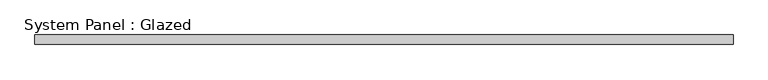
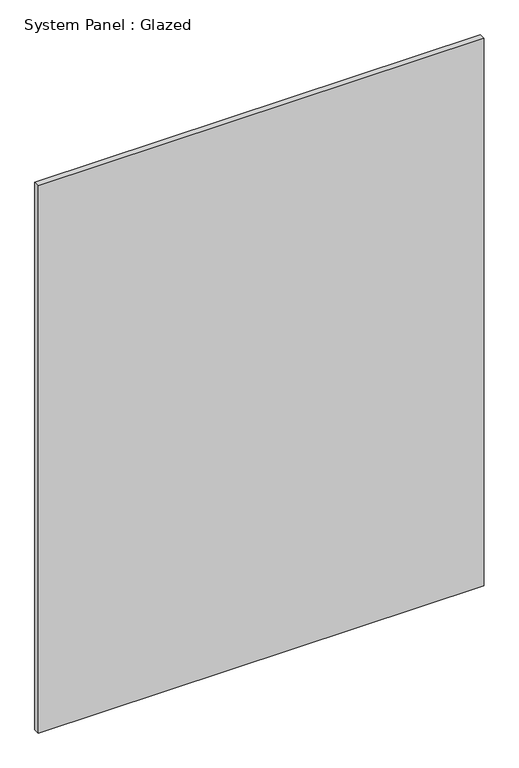
"""IFC4 building model written with IfcOpenShell, lengths in millimetres: plate geometry, System Panel : Glazed."""

from ifc_helpers import new_model, si_unit, origin, origin_with_axes, place, context, project, spatial, polyline, outline, extrude, source, transform, mapped, element, save


def system_panel_glazed_1fe62560(model_context):
    return source(origin(), model_context, "Body", "SweptSolid", [
        extrude(outline(polyline([(915.0000002, 24.5), (-915.0000002, 24.5), (-915.0000002, 49.5), (915.0000002, 49.5), (915.0000002, 24.5)])), origin_with_axes(), (0.0, 0.0, 1.0), 2375.0),
    ])


if __name__ == "__main__":
    model = new_model("IFC4")
    model_context = context("Model", 3, world=origin())
    ifc_project = project(units=[si_unit("LENGTHUNIT", "METRE", prefix="MILLI")], contexts=[model_context])
    site = spatial("IfcSite", under=ifc_project)
    building = spatial("IfcBuilding", under=site)
    placement = place(None, origin())
    system_panel_glazed_shape = system_panel_glazed_1fe62560(model_context)
    element("IfcPlate", 1, ObjectType="System Panel : Glazed", at=placement, inside=building, context=model_context, shape_type="MappedRepresentation", body=[
        mapped(system_panel_glazed_shape, transform((0.0, 0.0, 0.0), x_axis=(1.0, 0.0, 0.0), y_axis=(0.0, 1.0, 0.0), z_axis=(0.0, 0.0, 1.0))),
    ])
    save(model, "model.ifc")

# Revit data of these elements
# Element 1 (IfcPlate, "System Panel : Glazed")
#   Materials on its faces: "Glass"
# Materials
#   "Glass": class "Glass", colour RGB 218 227 224, transparency 0.85, Description = "Soda Lime Glass", Cost = 0
